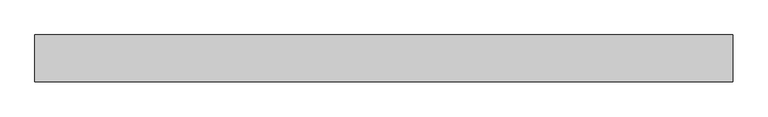
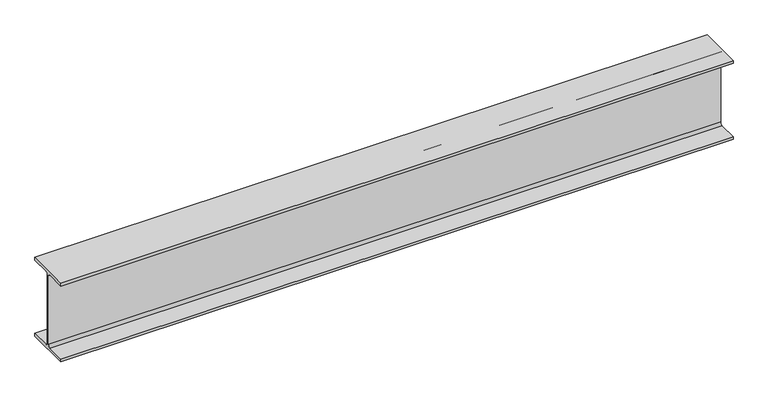
"""IFC4 building model written with IfcOpenShell, lengths in millimetres: beam geometry, Old_Steel Beam_H-KSD3502 : H_SB_ASB_H-350×175x7x11."""

from ifc_helpers import new_model, si_unit, point, frame, frame_2d, origin, place, context, project, spatial, polyline, circle_curve, trimmed, segment, composite_curve, outline, extrude, source, transform, mapped, element, save


def beam_7ca1c4d5(model_context):
    return source(origin(), model_context, "Body", "SweptSolid", [
        extrude(outline(composite_curve([segment(polyline([(82.5, -141.5), (82.5, -151.7), (-82.5, -151.7), (-82.5, -141.5), (-11.9, -141.5)]), True, "CONTINUOUS"), segment(trimmed(circle_curve(frame_2d((-11.9, -132.6)), 8.9), [point((-11.9, -141.5))], [point((-3.0, -132.6))], True, "CARTESIAN"), True, "CONTINUOUS"), segment(polyline([(-3.0, -132.6), (-3.0, 132.6)]), True, "CONTINUOUS"), segment(trimmed(circle_curve(frame_2d((-11.9, 132.6)), 8.9), [point((-3.0, 132.6))], [point((-11.9, 141.5))], True, "CARTESIAN"), True, "CONTINUOUS"), segment(polyline([(-11.9, 141.5), (-82.5, 141.5), (-82.5, 151.7), (82.5, 151.7), (82.5, 141.5), (11.9, 141.5)]), True, "CONTINUOUS"), segment(trimmed(circle_curve(frame_2d((11.9, 132.6)), 8.9), [point((11.9, 141.5))], [point((3.0, 132.6))], True, "CARTESIAN"), True, "CONTINUOUS"), segment(polyline([(3.0, 132.6), (3.0, -132.6)]), True, "CONTINUOUS"), segment(trimmed(circle_curve(frame_2d((11.9, -132.6)), 8.9), [point((3.0, -132.6))], [point((11.9, -141.5))], True, "CARTESIAN"), True, "CONTINUOUS"), segment(polyline([(11.9, -141.5), (82.5, -141.5)]), True, "CONTINUOUS")], self_intersect=False)), frame((-1295.7739051, 0.0, 0.0), z_axis=(1.0, 0.0, 0.0), x_axis=(0.0, 1.0, 0.0)), (0.0, 0.0, 1.0), 2456.2874909),
    ])


if __name__ == "__main__":
    model = new_model("IFC4")
    model_context = context("Model", 3, world=origin())
    ifc_project = project(units=[si_unit("LENGTHUNIT", "METRE", prefix="MILLI")], contexts=[model_context])
    site = spatial("IfcSite", under=ifc_project)
    building = spatial("IfcBuilding", under=site)
    placement = place(None, origin())
    beam_shape = beam_7ca1c4d5(model_context)
    element("IfcBeam", 1, ObjectType="Old_Steel Beam_H-KSD3502 : H_SB_ASB_H-350×175x7x11", at=placement, inside=building, context=model_context, shape_type="MappedRepresentation", body=[
        mapped(beam_shape, transform((0.0, 0.0, 0.0), x_axis=(1.0, 0.0, 0.0), y_axis=(0.0, 1.0, 0.0), z_axis=(0.0, 0.0, 1.0))),
    ])
    save(model, "model.ifc")

# Revit data of these elements
# Type "Old_Steel Beam_H-KSD3502 : H_SB_ASB_H-350×175x7x11"
#   Width = 17.5 cm
#   Web Thickness = 0.7 cm
#   Web Fillet = 1.4 cm
#   Warping Constant = 282290.0 cm⁶
#   Torsional Moment of Inertia = 19.4042 cm⁴
#   Torsional Modulus = 1.0 cm³
#   Section Area = 63.14 cm²
#   Plastic Modulus weak axis = 174.0 cm³
#   Plastic Modulus strong axis = 868.0 cm³
#   Perimeter = 1.36 m²/m
#   Nominal Weight = 49.60 kgf/m
#   Moment of Inertia weak axis = 984.00 cm⁴
#   Moment of Inertia strong axis = 13600.00 cm⁴
#   Height = 35.0 cm
#   Flange Thickness = 1.1 cm
#   Elastic Modulus weak axis = 112.0 cm³
#   Elastic Modulus strong axis = 775.0 cm³
#   Centroid Vertical = 17.5 cm
#   Centroid Horizontal = 8.75 cm
#   Length [instance default] = 1.5240 m
#   Structural Material [instance default] = Steel, 45-345
#   Assembly Code = ""
# Element 1 (IfcBeam, "Old_Steel Beam_H-KSD3502 : H_SB_ASB_H-350×175x7x11")
#   Structural Material = none
# Materials
#   "Steel, 45-345": class "Metal", colour RGB 189 187 185, transparency 0, Description = "Steel 345 MPa", Cost = 0
